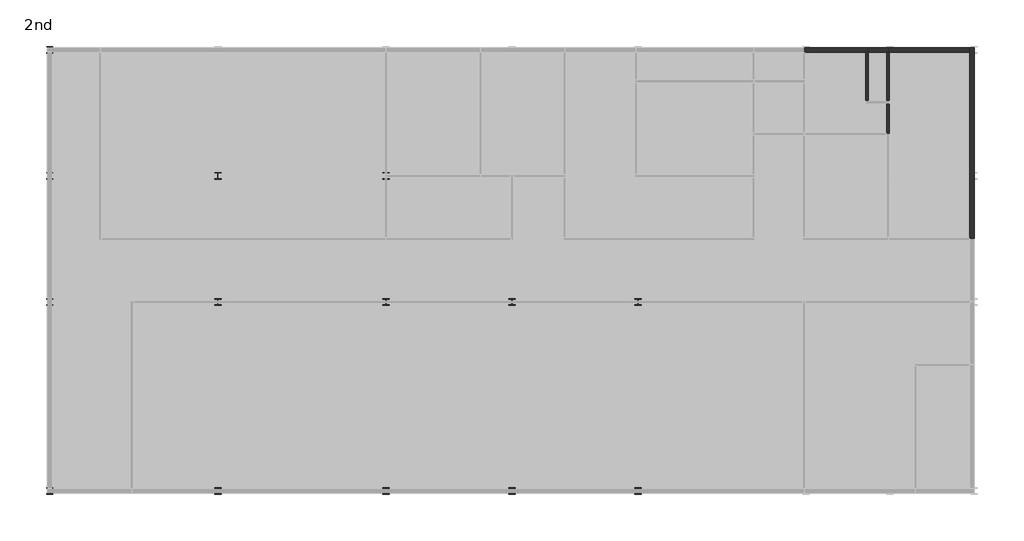
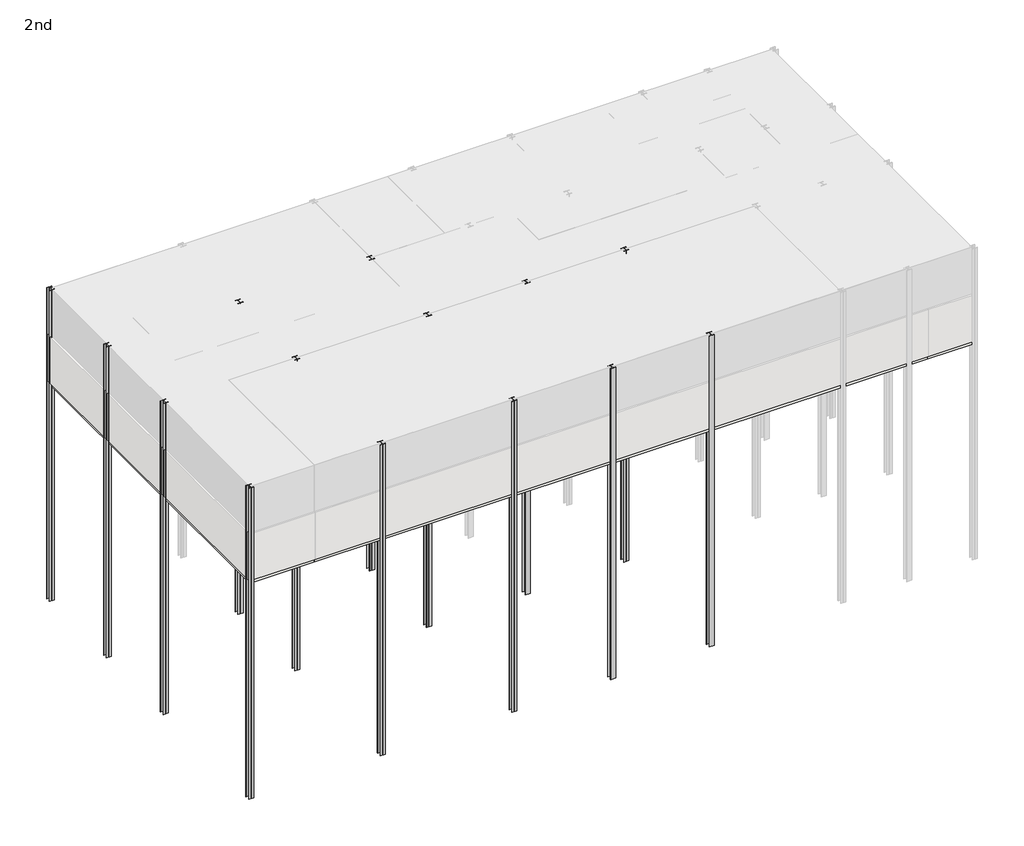
# One storey, part 2 of 3: 17 slabs, 14 columns, 7 walls.
"""IFC4 building model written with IfcOpenShell, lengths in millimetres."""

import ifcopenshell
import ifcopenshell.guid

model = None  # the IFC model being written
_history = None  # IfcOwnerHistory: only IFC2X3 demands one
_inside = {}  # id of a spatial element -> (the spatial element, [elements in it])
_under = {}  # id of a project, library or spatial element -> (it, [spatial elements below it])
_declared = {}  # id of a project -> (the project, [libraries it declares])
_typed = {}  # id of a type object -> (the type object, [elements of that type])
_made_of = {}  # id of a material, layer set ... -> (it, [elements and type objects made of it])


def new_model(schema):
    """Start an empty IFC model of exactly this schema.

    Asked for "IFC4X3", IfcOpenShell would pick the latest addendum, in which some entities
    have other attributes; the version numbers below select the first issue.
    IFC2X3 requires an IfcOwnerHistory on every rooted entity: one is made here for all.
    """
    global model, _history
    if schema == "IFC4X3":
        model = ifcopenshell.file(schema_version=(4, 3, 0, 0))
    else:
        model = ifcopenshell.file(schema=schema)
    _inside.clear()
    _under.clear()
    _declared.clear()
    _typed.clear()
    _made_of.clear()
    _history = None
    if model.schema == "IFC2X3":
        org = make("IfcOrganization", Name="unknown")
        user = make(
            "IfcPersonAndOrganization",
            ThePerson=make("IfcPerson", FamilyName="unknown"),
            TheOrganization=org,
        )
        app = make(
            "IfcApplication",
            ApplicationDeveloper=org,
            Version="unknown",
            ApplicationFullName="unknown",
            ApplicationIdentifier="unknown",
        )
        _history = make(
            "IfcOwnerHistory",
            OwningUser=user,
            OwningApplication=app,
            ChangeAction="ADDED",
            CreationDate=0,
        )
    return model


def make(cls, **values):
    """One entity of the class cls with the attributes given. An attribute that is None is left unset."""
    return model.create_entity(
        cls, **{name: value for name, value in values.items() if value is not None}
    )


def rooted(cls, **values):
    """An entity with a GlobalId (a new one), such as an element, a storey or a relation."""
    return make(cls, GlobalId=ifcopenshell.guid.new(), OwnerHistory=_history, **values)


def si_unit(unit_type, name, prefix=None):
    """IfcSIUnit, for example si_unit("LENGTHUNIT", "METRE", prefix="MILLI")."""
    return make("IfcSIUnit", UnitType=unit_type, Prefix=prefix, Name=name)


def assignment(units):
    """IfcUnitAssignment: the units of a project."""
    return None if units is None else make("IfcUnitAssignment", Units=units)


def point(xyz):
    """IfcCartesianPoint."""
    return None if xyz is None else make("IfcCartesianPoint", Coordinates=xyz)


def direction(xyz):
    """IfcDirection."""
    return None if xyz is None else make("IfcDirection", DirectionRatios=xyz)


def frame(location, z_axis=None, x_axis=None):
    """IfcAxis2Placement3D, a coordinate frame: its origin and axes. An axis left out is left unset."""
    return make(
        "IfcAxis2Placement3D",
        Location=point(location),
        Axis=direction(z_axis),
        RefDirection=direction(x_axis),
    )


def frame_2d(location, x_axis=None):
    """IfcAxis2Placement2D, a coordinate frame in the plane: its origin and x axis."""
    return make(
        "IfcAxis2Placement2D", Location=point(location), RefDirection=direction(x_axis)
    )


def origin():
    """The frame at (0, 0, 0) with its axes left unset."""
    return frame((0.0, 0.0, 0.0))


def origin_with_axes():
    """The frame at (0, 0, 0) with the z axis (0, 0, 1) and the x axis (1, 0, 0) written out."""
    return frame((0.0, 0.0, 0.0), z_axis=(0.0, 0.0, 1.0), x_axis=(1.0, 0.0, 0.0))


def place(relative_to, where):
    """IfcLocalPlacement: puts the frame where relative to a parent placement (None: the world)."""
    return make(
        "IfcLocalPlacement", PlacementRelTo=relative_to, RelativePlacement=where
    )


def context(
    kind, dimensions, precision=None, world=None, true_north=None, identifier=None
):
    """IfcGeometricRepresentationContext, for example the 3D "Model" context."""
    return make(
        "IfcGeometricRepresentationContext",
        ContextIdentifier=identifier,
        ContextType=kind,
        CoordinateSpaceDimension=dimensions,
        Precision=precision,
        WorldCoordinateSystem=world,
        TrueNorth=true_north,
    )


def project(units=None, contexts=None):
    """IfcProject with its units and contexts."""
    return rooted(
        "IfcProject",
        Name="project",
        RepresentationContexts=contexts,
        UnitsInContext=assignment(units),
    )


def spatial(cls, under=None, at=None, **own):
    """A site, building, storey or space (cls), placed at a placement, below another one or the project."""
    s = rooted(cls, ObjectPlacement=at, **own)
    if under is not None:
        _under.setdefault(under.id(), (under, []))[1].append(s)
    return s


def polyline(points):
    """IfcPolyline through the points."""
    return make("IfcPolyline", Points=[point(p) for p in points])


def circle_curve(where, radius):
    """IfcCircle in the frame where."""
    return make("IfcCircle", Position=where, Radius=radius)


def trimmed(basis, trim1, trim2, sense, master):
    """IfcTrimmedCurve: the piece of a basis curve between two trims."""
    return make(
        "IfcTrimmedCurve",
        BasisCurve=basis,
        Trim1=trim1,
        Trim2=trim2,
        SenseAgreement=sense,
        MasterRepresentation=master,
    )


def segment(curve, same_sense, transition):
    """IfcCompositeCurveSegment."""
    return make(
        "IfcCompositeCurveSegment",
        Transition=transition,
        SameSense=same_sense,
        ParentCurve=curve,
    )


def composite_curve(segments, self_intersect=None):
    """IfcCompositeCurve: segments joined end to end."""
    return make("IfcCompositeCurve", Segments=segments, SelfIntersect=self_intersect)


def outline(outer, holes=None, kind="AREA"):
    """IfcArbitraryClosedProfileDef: a profile drawn as a closed curve; with holes, ...WithVoids."""
    if holes is None:
        return make("IfcArbitraryClosedProfileDef", ProfileType=kind, OuterCurve=outer)
    return make(
        "IfcArbitraryProfileDefWithVoids",
        ProfileType=kind,
        OuterCurve=outer,
        InnerCurves=holes,
    )


def extrude(swept, where, along, depth):
    """IfcExtrudedAreaSolid: the profile swept, set in the frame where, extruded along a direction by depth."""
    return make(
        "IfcExtrudedAreaSolid",
        SweptArea=swept,
        Position=where,
        ExtrudedDirection=direction(along),
        Depth=depth,
    )


def faces_of(points, faces, orient=None, outer=None):
    """IfcFace entities. A face is a list of loops; a loop is a list of indices into points, from 0.

    orient and outer hold one flag for each loop. By default every Orientation is true, the
    first loop of a face is its IfcFaceOuterBound and the others are IfcFaceBound.
    """
    made = []
    for i, loops in enumerate(faces):
        bounds = []
        for j, loop in enumerate(loops):
            is_outer = j == 0 if outer is None else outer[i][j]
            bounds.append(
                make(
                    "IfcFaceOuterBound" if is_outer else "IfcFaceBound",
                    Bound=make("IfcPolyLoop", Polygon=[points[k] for k in loop]),
                    Orientation=True if orient is None else orient[i][j],
                )
            )
        made.append(make("IfcFace", Bounds=bounds))
    return made


def faceted_brep(points, faces, orient=None, outer=None, voids=None):
    """IfcFacetedBrep: a solid bounded by flat faces; with voids (closed shells), ...WithVoids."""
    shared = [point(p) for p in points]
    hull = make("IfcClosedShell", CfsFaces=faces_of(shared, faces, orient, outer))
    if voids is None:
        return make("IfcFacetedBrep", Outer=hull)
    return make(
        "IfcFacetedBrepWithVoids",
        Outer=hull,
        Voids=[
            make(cls, CfsFaces=faces_of(shared, fs, o, b)) for cls, fs, o, b in voids
        ],
    )


def shape(context_of_items, identifier, shape_type, items):
    """IfcShapeRepresentation: the items that make up one representation, for example the "Body"."""
    return make(
        "IfcShapeRepresentation",
        ContextOfItems=context_of_items,
        RepresentationIdentifier=identifier,
        RepresentationType=shape_type,
        Items=items,
    )


def made_of(thing, what):
    """Note that an element or type object is made of a material, layer set ...; save() writes the relation."""
    if what is not None:
        _made_of.setdefault(what.id(), (what, []))[1].append(thing)
    return thing


def element(
    cls,
    number,
    at=None,
    inside=None,
    cuts=None,
    type_object=None,
    material=None,
    context=None,
    identifier="Body",
    shape_type=None,
    held_by="IfcProductDefinitionShape",
    body=None,
    shapes=None,
    **own,
):
    """One element of the class cls, such as IfcWall. Its Tag is "e" and its number.

    at: its placement. inside: the storey or other place that contains it. cuts: it is an
    opening in that element (IfcRelVoidsElement). A single representation is given by context,
    identifier, shape_type and body (its items); several are given by shapes. held_by: the class
    of the entity that holds the representations. save() writes the other relations.
    """
    e = rooted(cls, Tag="e%d" % number, ObjectPlacement=at, **own)
    if body is not None:
        shapes = [shape(context, identifier, shape_type, body)]
    if shapes is not None:
        e.Representation = make(held_by, Representations=shapes)
    if inside is not None:
        _inside.setdefault(inside.id(), (inside, []))[1].append(e)
    if cuts is not None:
        rooted(
            "IfcRelVoidsElement", RelatingBuildingElement=cuts, RelatedOpeningElement=e
        )
    if type_object is not None:
        _typed.setdefault(type_object.id(), (type_object, []))[1].append(e)
    return made_of(e, material)


def aggregate(whole, parts):
    """IfcRelAggregates: a whole, such as a stair, and the parts it consists of."""
    return rooted("IfcRelAggregates", RelatingObject=whole, RelatedObjects=parts)


def save(model, path):
    """Write the relations noted so far, then the file.

    IfcRelAggregates (storeys below a building ...), IfcRelContainedInSpatialStructure (elements
    in a storey), IfcRelDefinesByType, IfcRelAssociatesMaterial and IfcRelDeclares: one each for
    every whole, place, type object, material and project.
    """
    for whole, parts in _under.values():
        aggregate(whole, parts)
    for where, things in _inside.values():
        rooted(
            "IfcRelContainedInSpatialStructure",
            RelatedElements=things,
            RelatingStructure=where,
        )
    for kind, things in _typed.values():
        rooted("IfcRelDefinesByType", RelatedObjects=things, RelatingType=kind)
    for what, things in _made_of.values():
        rooted("IfcRelAssociatesMaterial", RelatedObjects=things, RelatingMaterial=what)
    for by, libraries in _declared.values():
        rooted("IfcRelDeclares", RelatingContext=by, RelatedDefinitions=libraries)
    model.write(path)


model = new_model("IFC4")

# Units and contexts
model_context = context("Model", 3, world=origin())
ifc_project = project(units=[si_unit("LENGTHUNIT", "METRE", prefix="MILLI")], contexts=[model_context])

# Site, building, storey
site = spatial("IfcSite", under=ifc_project)
building = spatial("IfcBuilding", under=site)
storey = spatial("IfcBuildingStorey", under=building, Name="2nd", Elevation=14000.0)

# Columns
placement = place(None, origin())
element("IfcColumn", 1, ObjectType="UC-Universal Columns-Column : UC305x305x97", at=placement, inside=storey, context=model_context, shape_type="SweptSolid", body=[
    extrude(outline(composite_curve([segment(polyline([(156266.7520501, 152169.7081198), (156266.7520501, 152154.3081198), (156134.2520501, 152154.3081198)]), True, "CONTINUOUS"), segment(trimmed(circle_curve(frame_2d((156134.2520501, 152139.1081198)), 15.2), [point((156134.2520501, 152154.3081198))], [point((156119.0520501, 152139.1081198))], True, "CARTESIAN"), True, "CONTINUOUS"), segment(polyline([(156119.0520501, 152139.1081198), (156119.0520501, 151892.4081198)]), True, "CONTINUOUS"), segment(trimmed(circle_curve(frame_2d((156134.2520501, 151892.4081198)), 15.2), [point((156119.0520501, 151892.4081198))], [point((156134.2520501, 151877.2081198))], True, "CARTESIAN"), True, "CONTINUOUS"), segment(polyline([(156134.2520501, 151877.2081198), (156266.7520501, 151877.2081198), (156266.7520501, 151861.8081198), (155961.4520501, 151861.8081198), (155961.4520501, 151877.2081198), (156093.9520501, 151877.2081198)]), True, "CONTINUOUS"), segment(trimmed(circle_curve(frame_2d((156093.9520501, 151892.4081198)), 15.2), [point((156093.9520501, 151877.2081198))], [point((156109.1520501, 151892.4081198))], True, "CARTESIAN"), True, "CONTINUOUS"), segment(polyline([(156109.1520501, 151892.4081198), (156109.1520501, 152139.1081198)]), True, "CONTINUOUS"), segment(trimmed(circle_curve(frame_2d((156093.9520501, 152139.1081198)), 15.2), [point((156109.1520501, 152139.1081198))], [point((156093.9520501, 152154.3081198))], True, "CARTESIAN"), True, "CONTINUOUS"), segment(polyline([(156093.9520501, 152154.3081198), (155961.4520501, 152154.3081198), (155961.4520501, 152169.7081198), (156266.7520501, 152169.7081198)]), True, "CONTINUOUS")], self_intersect=False)), origin_with_axes(), (0.0, 0.0, 1.0), 20000.0),
])
element("IfcColumn", 2, ObjectType="UC-Universal Columns-Column : UC305x305x97", at=placement, inside=storey, context=model_context, shape_type="SweptSolid", body=[
    extrude(outline(composite_curve([segment(polyline([(156266.7520501, 146169.7081198), (156266.7520501, 146154.3081198), (156134.2520501, 146154.3081198)]), True, "CONTINUOUS"), segment(trimmed(circle_curve(frame_2d((156134.2520501, 146139.1081198)), 15.2), [point((156134.2520501, 146154.3081198))], [point((156119.0520501, 146139.1081198))], True, "CARTESIAN"), True, "CONTINUOUS"), segment(polyline([(156119.0520501, 146139.1081198), (156119.0520501, 145892.4081198)]), True, "CONTINUOUS"), segment(trimmed(circle_curve(frame_2d((156134.2520501, 145892.4081198)), 15.2), [point((156119.0520501, 145892.4081198))], [point((156134.2520501, 145877.2081198))], True, "CARTESIAN"), True, "CONTINUOUS"), segment(polyline([(156134.2520501, 145877.2081198), (156266.7520501, 145877.2081198), (156266.7520501, 145861.8081198), (155961.4520501, 145861.8081198), (155961.4520501, 145877.2081198), (156093.9520501, 145877.2081198)]), True, "CONTINUOUS"), segment(trimmed(circle_curve(frame_2d((156093.9520501, 145892.4081198)), 15.2), [point((156093.9520501, 145877.2081198))], [point((156109.1520501, 145892.4081198))], True, "CARTESIAN"), True, "CONTINUOUS"), segment(polyline([(156109.1520501, 145892.4081198), (156109.1520501, 146139.1081198)]), True, "CONTINUOUS"), segment(trimmed(circle_curve(frame_2d((156093.9520501, 146139.1081198)), 15.2), [point((156109.1520501, 146139.1081198))], [point((156093.9520501, 146154.3081198))], True, "CARTESIAN"), True, "CONTINUOUS"), segment(polyline([(156093.9520501, 146154.3081198), (155961.4520501, 146154.3081198), (155961.4520501, 146169.7081198), (156266.7520501, 146169.7081198)]), True, "CONTINUOUS")], self_intersect=False)), origin_with_axes(), (0.0, 0.0, 1.0), 20000.0),
])
element("IfcColumn", 3, ObjectType="UC-Universal Columns-Column : UC305x305x97", at=placement, inside=storey, context=model_context, shape_type="SweptSolid", body=[
    extrude(outline(composite_curve([segment(polyline([(156266.7520501, 140169.7081198), (156266.7520501, 140154.3081198), (156134.2520501, 140154.3081198)]), True, "CONTINUOUS"), segment(trimmed(circle_curve(frame_2d((156134.2520501, 140139.1081198)), 15.2), [point((156134.2520501, 140154.3081198))], [point((156119.0520501, 140139.1081198))], True, "CARTESIAN"), True, "CONTINUOUS"), segment(polyline([(156119.0520501, 140139.1081198), (156119.0520501, 139892.4081198)]), True, "CONTINUOUS"), segment(trimmed(circle_curve(frame_2d((156134.2520501, 139892.4081198)), 15.2), [point((156119.0520501, 139892.4081198))], [point((156134.2520501, 139877.2081198))], True, "CARTESIAN"), True, "CONTINUOUS"), segment(polyline([(156134.2520501, 139877.2081198), (156266.7520501, 139877.2081198), (156266.7520501, 139861.8081198), (155961.4520501, 139861.8081198), (155961.4520501, 139877.2081198), (156093.9520501, 139877.2081198)]), True, "CONTINUOUS"), segment(trimmed(circle_curve(frame_2d((156093.9520501, 139892.4081198)), 15.2), [point((156093.9520501, 139877.2081198))], [point((156109.1520501, 139892.4081198))], True, "CARTESIAN"), True, "CONTINUOUS"), segment(polyline([(156109.1520501, 139892.4081198), (156109.1520501, 140139.1081198)]), True, "CONTINUOUS"), segment(trimmed(circle_curve(frame_2d((156093.9520501, 140139.1081198)), 15.2), [point((156109.1520501, 140139.1081198))], [point((156093.9520501, 140154.3081198))], True, "CARTESIAN"), True, "CONTINUOUS"), segment(polyline([(156093.9520501, 140154.3081198), (155961.4520501, 140154.3081198), (155961.4520501, 140169.7081198), (156266.7520501, 140169.7081198)]), True, "CONTINUOUS")], self_intersect=False)), origin_with_axes(), (0.0, 0.0, 1.0), 20000.0),
])
element("IfcColumn", 4, ObjectType="UC-Universal Columns-Column : UC305x305x97", at=placement, inside=storey, context=model_context, shape_type="SweptSolid", body=[
    extrude(outline(composite_curve([segment(polyline([(156266.7520501, 131169.7081198), (156266.7520501, 131154.3081198), (156134.2520501, 131154.3081198)]), True, "CONTINUOUS"), segment(trimmed(circle_curve(frame_2d((156134.2520501, 131139.1081198)), 15.2), [point((156134.2520501, 131154.3081198))], [point((156119.0520501, 131139.1081198))], True, "CARTESIAN"), True, "CONTINUOUS"), segment(polyline([(156119.0520501, 131139.1081198), (156119.0520501, 130892.4081198)]), True, "CONTINUOUS"), segment(trimmed(circle_curve(frame_2d((156134.2520501, 130892.4081198)), 15.2), [point((156119.0520501, 130892.4081198))], [point((156134.2520501, 130877.2081198))], True, "CARTESIAN"), True, "CONTINUOUS"), segment(polyline([(156134.2520501, 130877.2081198), (156266.7520501, 130877.2081198), (156266.7520501, 130861.8081198), (155961.4520501, 130861.8081198), (155961.4520501, 130877.2081198), (156093.9520501, 130877.2081198)]), True, "CONTINUOUS"), segment(trimmed(circle_curve(frame_2d((156093.9520501, 130892.4081198)), 15.2), [point((156093.9520501, 130877.2081198))], [point((156109.1520501, 130892.4081198))], True, "CARTESIAN"), True, "CONTINUOUS"), segment(polyline([(156109.1520501, 130892.4081198), (156109.1520501, 131139.1081198)]), True, "CONTINUOUS"), segment(trimmed(circle_curve(frame_2d((156093.9520501, 131139.1081198)), 15.2), [point((156109.1520501, 131139.1081198))], [point((156093.9520501, 131154.3081198))], True, "CARTESIAN"), True, "CONTINUOUS"), segment(polyline([(156093.9520501, 131154.3081198), (155961.4520501, 131154.3081198), (155961.4520501, 131169.7081198), (156266.7520501, 131169.7081198)]), True, "CONTINUOUS")], self_intersect=False)), origin_with_axes(), (0.0, 0.0, 1.0), 20000.0),
])
element("IfcColumn", 5, ObjectType="UC-Universal Columns-Column : UC305x305x97", at=placement, inside=storey, context=model_context, shape_type="SweptSolid", body=[
    extrude(outline(composite_curve([segment(polyline([(164266.7520501, 146169.7081198), (164266.7520501, 146154.3081198), (164134.2520501, 146154.3081198)]), True, "CONTINUOUS"), segment(trimmed(circle_curve(frame_2d((164134.2520501, 146139.1081198)), 15.2), [point((164134.2520501, 146154.3081198))], [point((164119.0520501, 146139.1081198))], True, "CARTESIAN"), True, "CONTINUOUS"), segment(polyline([(164119.0520501, 146139.1081198), (164119.0520501, 145892.4081198)]), True, "CONTINUOUS"), segment(trimmed(circle_curve(frame_2d((164134.2520501, 145892.4081198)), 15.2), [point((164119.0520501, 145892.4081198))], [point((164134.2520501, 145877.2081198))], True, "CARTESIAN"), True, "CONTINUOUS"), segment(polyline([(164134.2520501, 145877.2081198), (164266.7520501, 145877.2081198), (164266.7520501, 145861.8081198), (163961.4520501, 145861.8081198), (163961.4520501, 145877.2081198), (164093.9520501, 145877.2081198)]), True, "CONTINUOUS"), segment(trimmed(circle_curve(frame_2d((164093.9520501, 145892.4081198)), 15.2), [point((164093.9520501, 145877.2081198))], [point((164109.1520501, 145892.4081198))], True, "CARTESIAN"), True, "CONTINUOUS"), segment(polyline([(164109.1520501, 145892.4081198), (164109.1520501, 146139.1081198)]), True, "CONTINUOUS"), segment(trimmed(circle_curve(frame_2d((164093.9520501, 146139.1081198)), 15.2), [point((164109.1520501, 146139.1081198))], [point((164093.9520501, 146154.3081198))], True, "CARTESIAN"), True, "CONTINUOUS"), segment(polyline([(164093.9520501, 146154.3081198), (163961.4520501, 146154.3081198), (163961.4520501, 146169.7081198), (164266.7520501, 146169.7081198)]), True, "CONTINUOUS")], self_intersect=False)), origin_with_axes(), (0.0, 0.0, 1.0), 20000.0),
])
element("IfcColumn", 6, ObjectType="UC-Universal Columns-Column : UC305x305x97", at=placement, inside=storey, context=model_context, shape_type="SweptSolid", body=[
    extrude(outline(composite_curve([segment(polyline([(164266.7520501, 140169.7081198), (164266.7520501, 140154.3081198), (164134.2520501, 140154.3081198)]), True, "CONTINUOUS"), segment(trimmed(circle_curve(frame_2d((164134.2520501, 140139.1081198)), 15.2), [point((164134.2520501, 140154.3081198))], [point((164119.0520501, 140139.1081198))], True, "CARTESIAN"), True, "CONTINUOUS"), segment(polyline([(164119.0520501, 140139.1081198), (164119.0520501, 139892.4081198)]), True, "CONTINUOUS"), segment(trimmed(circle_curve(frame_2d((164134.2520501, 139892.4081198)), 15.2), [point((164119.0520501, 139892.4081198))], [point((164134.2520501, 139877.2081198))], True, "CARTESIAN"), True, "CONTINUOUS"), segment(polyline([(164134.2520501, 139877.2081198), (164266.7520501, 139877.2081198), (164266.7520501, 139861.8081198), (163961.4520501, 139861.8081198), (163961.4520501, 139877.2081198), (164093.9520501, 139877.2081198)]), True, "CONTINUOUS"), segment(trimmed(circle_curve(frame_2d((164093.9520501, 139892.4081198)), 15.2), [point((164093.9520501, 139877.2081198))], [point((164109.1520501, 139892.4081198))], True, "CARTESIAN"), True, "CONTINUOUS"), segment(polyline([(164109.1520501, 139892.4081198), (164109.1520501, 140139.1081198)]), True, "CONTINUOUS"), segment(trimmed(circle_curve(frame_2d((164093.9520501, 140139.1081198)), 15.2), [point((164109.1520501, 140139.1081198))], [point((164093.9520501, 140154.3081198))], True, "CARTESIAN"), True, "CONTINUOUS"), segment(polyline([(164093.9520501, 140154.3081198), (163961.4520501, 140154.3081198), (163961.4520501, 140169.7081198), (164266.7520501, 140169.7081198)]), True, "CONTINUOUS")], self_intersect=False)), origin_with_axes(), (0.0, 0.0, 1.0), 20000.0),
])
element("IfcColumn", 7, ObjectType="UC-Universal Columns-Column : UC305x305x97", at=placement, inside=storey, context=model_context, shape_type="SweptSolid", body=[
    extrude(outline(composite_curve([segment(polyline([(164266.7520501, 131169.7081198), (164266.7520501, 131154.3081198), (164134.2520501, 131154.3081198)]), True, "CONTINUOUS"), segment(trimmed(circle_curve(frame_2d((164134.2520501, 131139.1081198)), 15.2), [point((164134.2520501, 131154.3081198))], [point((164119.0520501, 131139.1081198))], True, "CARTESIAN"), True, "CONTINUOUS"), segment(polyline([(164119.0520501, 131139.1081198), (164119.0520501, 130892.4081198)]), True, "CONTINUOUS"), segment(trimmed(circle_curve(frame_2d((164134.2520501, 130892.4081198)), 15.2), [point((164119.0520501, 130892.4081198))], [point((164134.2520501, 130877.2081198))], True, "CARTESIAN"), True, "CONTINUOUS"), segment(polyline([(164134.2520501, 130877.2081198), (164266.7520501, 130877.2081198), (164266.7520501, 130861.8081198), (163961.4520501, 130861.8081198), (163961.4520501, 130877.2081198), (164093.9520501, 130877.2081198)]), True, "CONTINUOUS"), segment(trimmed(circle_curve(frame_2d((164093.9520501, 130892.4081198)), 15.2), [point((164093.9520501, 130877.2081198))], [point((164109.1520501, 130892.4081198))], True, "CARTESIAN"), True, "CONTINUOUS"), segment(polyline([(164109.1520501, 130892.4081198), (164109.1520501, 131139.1081198)]), True, "CONTINUOUS"), segment(trimmed(circle_curve(frame_2d((164093.9520501, 131139.1081198)), 15.2), [point((164109.1520501, 131139.1081198))], [point((164093.9520501, 131154.3081198))], True, "CARTESIAN"), True, "CONTINUOUS"), segment(polyline([(164093.9520501, 131154.3081198), (163961.4520501, 131154.3081198), (163961.4520501, 131169.7081198), (164266.7520501, 131169.7081198)]), True, "CONTINUOUS")], self_intersect=False)), origin_with_axes(), (0.0, 0.0, 1.0), 20000.0),
])
element("IfcColumn", 8, ObjectType="UC-Universal Columns-Column : UC305x305x97", at=placement, inside=storey, context=model_context, shape_type="SweptSolid", body=[
    extrude(outline(composite_curve([segment(polyline([(172266.7520501, 146169.7081198), (172266.7520501, 146154.3081198), (172134.2520501, 146154.3081198)]), True, "CONTINUOUS"), segment(trimmed(circle_curve(frame_2d((172134.2520501, 146139.1081198)), 15.2), [point((172134.2520501, 146154.3081198))], [point((172119.0520501, 146139.1081198))], True, "CARTESIAN"), True, "CONTINUOUS"), segment(polyline([(172119.0520501, 146139.1081198), (172119.0520501, 145892.4081198)]), True, "CONTINUOUS"), segment(trimmed(circle_curve(frame_2d((172134.2520501, 145892.4081198)), 15.2), [point((172119.0520501, 145892.4081198))], [point((172134.2520501, 145877.2081198))], True, "CARTESIAN"), True, "CONTINUOUS"), segment(polyline([(172134.2520501, 145877.2081198), (172266.7520501, 145877.2081198), (172266.7520501, 145861.8081198), (171961.4520501, 145861.8081198), (171961.4520501, 145877.2081198), (172093.9520501, 145877.2081198)]), True, "CONTINUOUS"), segment(trimmed(circle_curve(frame_2d((172093.9520501, 145892.4081198)), 15.2), [point((172093.9520501, 145877.2081198))], [point((172109.1520501, 145892.4081198))], True, "CARTESIAN"), True, "CONTINUOUS"), segment(polyline([(172109.1520501, 145892.4081198), (172109.1520501, 146139.1081198)]), True, "CONTINUOUS"), segment(trimmed(circle_curve(frame_2d((172093.9520501, 146139.1081198)), 15.2), [point((172109.1520501, 146139.1081198))], [point((172093.9520501, 146154.3081198))], True, "CARTESIAN"), True, "CONTINUOUS"), segment(polyline([(172093.9520501, 146154.3081198), (171961.4520501, 146154.3081198), (171961.4520501, 146169.7081198), (172266.7520501, 146169.7081198)]), True, "CONTINUOUS")], self_intersect=False)), origin_with_axes(), (0.0, 0.0, 1.0), 20000.0),
])
element("IfcColumn", 9, ObjectType="UC-Universal Columns-Column : UC305x305x97", at=placement, inside=storey, context=model_context, shape_type="SweptSolid", body=[
    extrude(outline(composite_curve([segment(polyline([(172266.7520501, 140169.7081198), (172266.7520501, 140154.3081198), (172134.2520501, 140154.3081198)]), True, "CONTINUOUS"), segment(trimmed(circle_curve(frame_2d((172134.2520501, 140139.1081198)), 15.2), [point((172134.2520501, 140154.3081198))], [point((172119.0520501, 140139.1081198))], True, "CARTESIAN"), True, "CONTINUOUS"), segment(polyline([(172119.0520501, 140139.1081198), (172119.0520501, 139892.4081198)]), True, "CONTINUOUS"), segment(trimmed(circle_curve(frame_2d((172134.2520501, 139892.4081198)), 15.2), [point((172119.0520501, 139892.4081198))], [point((172134.2520501, 139877.2081198))], True, "CARTESIAN"), True, "CONTINUOUS"), segment(polyline([(172134.2520501, 139877.2081198), (172266.7520501, 139877.2081198), (172266.7520501, 139861.8081198), (171961.4520501, 139861.8081198), (171961.4520501, 139877.2081198), (172093.9520501, 139877.2081198)]), True, "CONTINUOUS"), segment(trimmed(circle_curve(frame_2d((172093.9520501, 139892.4081198)), 15.2), [point((172093.9520501, 139877.2081198))], [point((172109.1520501, 139892.4081198))], True, "CARTESIAN"), True, "CONTINUOUS"), segment(polyline([(172109.1520501, 139892.4081198), (172109.1520501, 140139.1081198)]), True, "CONTINUOUS"), segment(trimmed(circle_curve(frame_2d((172093.9520501, 140139.1081198)), 15.2), [point((172109.1520501, 140139.1081198))], [point((172093.9520501, 140154.3081198))], True, "CARTESIAN"), True, "CONTINUOUS"), segment(polyline([(172093.9520501, 140154.3081198), (171961.4520501, 140154.3081198), (171961.4520501, 140169.7081198), (172266.7520501, 140169.7081198)]), True, "CONTINUOUS")], self_intersect=False)), origin_with_axes(), (0.0, 0.0, 1.0), 20000.0),
])
element("IfcColumn", 10, ObjectType="UC-Universal Columns-Column : UC305x305x97", at=placement, inside=storey, context=model_context, shape_type="SweptSolid", body=[
    extrude(outline(composite_curve([segment(polyline([(172266.7520501, 131169.7081198), (172266.7520501, 131154.3081198), (172134.2520501, 131154.3081198)]), True, "CONTINUOUS"), segment(trimmed(circle_curve(frame_2d((172134.2520501, 131139.1081198)), 15.2), [point((172134.2520501, 131154.3081198))], [point((172119.0520501, 131139.1081198))], True, "CARTESIAN"), True, "CONTINUOUS"), segment(polyline([(172119.0520501, 131139.1081198), (172119.0520501, 130892.4081198)]), True, "CONTINUOUS"), segment(trimmed(circle_curve(frame_2d((172134.2520501, 130892.4081198)), 15.2), [point((172119.0520501, 130892.4081198))], [point((172134.2520501, 130877.2081198))], True, "CARTESIAN"), True, "CONTINUOUS"), segment(polyline([(172134.2520501, 130877.2081198), (172266.7520501, 130877.2081198), (172266.7520501, 130861.8081198), (171961.4520501, 130861.8081198), (171961.4520501, 130877.2081198), (172093.9520501, 130877.2081198)]), True, "CONTINUOUS"), segment(trimmed(circle_curve(frame_2d((172093.9520501, 130892.4081198)), 15.2), [point((172093.9520501, 130877.2081198))], [point((172109.1520501, 130892.4081198))], True, "CARTESIAN"), True, "CONTINUOUS"), segment(polyline([(172109.1520501, 130892.4081198), (172109.1520501, 131139.1081198)]), True, "CONTINUOUS"), segment(trimmed(circle_curve(frame_2d((172093.9520501, 131139.1081198)), 15.2), [point((172109.1520501, 131139.1081198))], [point((172093.9520501, 131154.3081198))], True, "CARTESIAN"), True, "CONTINUOUS"), segment(polyline([(172093.9520501, 131154.3081198), (171961.4520501, 131154.3081198), (171961.4520501, 131169.7081198), (172266.7520501, 131169.7081198)]), True, "CONTINUOUS")], self_intersect=False)), origin_with_axes(), (0.0, 0.0, 1.0), 20000.0),
])
element("IfcColumn", 11, ObjectType="UC-Universal Columns-Column : UC305x305x97", at=placement, inside=storey, context=model_context, shape_type="SweptSolid", body=[
    extrude(outline(composite_curve([segment(polyline([(178266.7520501, 140169.7081198), (178266.7520501, 140154.3081198), (178134.2520501, 140154.3081198)]), True, "CONTINUOUS"), segment(trimmed(circle_curve(frame_2d((178134.2520501, 140139.1081198)), 15.2), [point((178134.2520501, 140154.3081198))], [point((178119.0520501, 140139.1081198))], True, "CARTESIAN"), True, "CONTINUOUS"), segment(polyline([(178119.0520501, 140139.1081198), (178119.0520501, 139892.4081198)]), True, "CONTINUOUS"), segment(trimmed(circle_curve(frame_2d((178134.2520501, 139892.4081198)), 15.2), [point((178119.0520501, 139892.4081198))], [point((178134.2520501, 139877.2081198))], True, "CARTESIAN"), True, "CONTINUOUS"), segment(polyline([(178134.2520501, 139877.2081198), (178266.7520501, 139877.2081198), (178266.7520501, 139861.8081198), (177961.4520501, 139861.8081198), (177961.4520501, 139877.2081198), (178093.9520501, 139877.2081198)]), True, "CONTINUOUS"), segment(trimmed(circle_curve(frame_2d((178093.9520501, 139892.4081198)), 15.2), [point((178093.9520501, 139877.2081198))], [point((178109.1520501, 139892.4081198))], True, "CARTESIAN"), True, "CONTINUOUS"), segment(polyline([(178109.1520501, 139892.4081198), (178109.1520501, 140139.1081198)]), True, "CONTINUOUS"), segment(trimmed(circle_curve(frame_2d((178093.9520501, 140139.1081198)), 15.2), [point((178109.1520501, 140139.1081198))], [point((178093.9520501, 140154.3081198))], True, "CARTESIAN"), True, "CONTINUOUS"), segment(polyline([(178093.9520501, 140154.3081198), (177961.4520501, 140154.3081198), (177961.4520501, 140169.7081198), (178266.7520501, 140169.7081198)]), True, "CONTINUOUS")], self_intersect=False)), origin_with_axes(), (0.0, 0.0, 1.0), 20000.0),
])
element("IfcColumn", 12, ObjectType="UC-Universal Columns-Column : UC305x305x97", at=placement, inside=storey, context=model_context, shape_type="SweptSolid", body=[
    extrude(outline(composite_curve([segment(polyline([(178266.7520501, 131169.7081198), (178266.7520501, 131154.3081198), (178134.2520501, 131154.3081198)]), True, "CONTINUOUS"), segment(trimmed(circle_curve(frame_2d((178134.2520501, 131139.1081198)), 15.2), [point((178134.2520501, 131154.3081198))], [point((178119.0520501, 131139.1081198))], True, "CARTESIAN"), True, "CONTINUOUS"), segment(polyline([(178119.0520501, 131139.1081198), (178119.0520501, 130892.4081198)]), True, "CONTINUOUS"), segment(trimmed(circle_curve(frame_2d((178134.2520501, 130892.4081198)), 15.2), [point((178119.0520501, 130892.4081198))], [point((178134.2520501, 130877.2081198))], True, "CARTESIAN"), True, "CONTINUOUS"), segment(polyline([(178134.2520501, 130877.2081198), (178266.7520501, 130877.2081198), (178266.7520501, 130861.8081198), (177961.4520501, 130861.8081198), (177961.4520501, 130877.2081198), (178093.9520501, 130877.2081198)]), True, "CONTINUOUS"), segment(trimmed(circle_curve(frame_2d((178093.9520501, 130892.4081198)), 15.2), [point((178093.9520501, 130877.2081198))], [point((178109.1520501, 130892.4081198))], True, "CARTESIAN"), True, "CONTINUOUS"), segment(polyline([(178109.1520501, 130892.4081198), (178109.1520501, 131139.1081198)]), True, "CONTINUOUS"), segment(trimmed(circle_curve(frame_2d((178093.9520501, 131139.1081198)), 15.2), [point((178109.1520501, 131139.1081198))], [point((178093.9520501, 131154.3081198))], True, "CARTESIAN"), True, "CONTINUOUS"), segment(polyline([(178093.9520501, 131154.3081198), (177961.4520501, 131154.3081198), (177961.4520501, 131169.7081198), (178266.7520501, 131169.7081198)]), True, "CONTINUOUS")], self_intersect=False)), origin_with_axes(), (0.0, 0.0, 1.0), 20000.0),
])
element("IfcColumn", 13, ObjectType="UC-Universal Columns-Column : UC305x305x97", at=placement, inside=storey, context=model_context, shape_type="SweptSolid", body=[
    extrude(outline(composite_curve([segment(polyline([(184266.7520501, 140169.7081198), (184266.7520501, 140154.3081198), (184134.2520501, 140154.3081198)]), True, "CONTINUOUS"), segment(trimmed(circle_curve(frame_2d((184134.2520501, 140139.1081198)), 15.2), [point((184134.2520501, 140154.3081198))], [point((184119.0520501, 140139.1081198))], True, "CARTESIAN"), True, "CONTINUOUS"), segment(polyline([(184119.0520501, 140139.1081198), (184119.0520501, 139892.4081198)]), True, "CONTINUOUS"), segment(trimmed(circle_curve(frame_2d((184134.2520501, 139892.4081198)), 15.2), [point((184119.0520501, 139892.4081198))], [point((184134.2520501, 139877.2081198))], True, "CARTESIAN"), True, "CONTINUOUS"), segment(polyline([(184134.2520501, 139877.2081198), (184266.7520501, 139877.2081198), (184266.7520501, 139861.8081198), (183961.4520501, 139861.8081198), (183961.4520501, 139877.2081198), (184093.9520501, 139877.2081198)]), True, "CONTINUOUS"), segment(trimmed(circle_curve(frame_2d((184093.9520501, 139892.4081198)), 15.2), [point((184093.9520501, 139877.2081198))], [point((184109.1520501, 139892.4081198))], True, "CARTESIAN"), True, "CONTINUOUS"), segment(polyline([(184109.1520501, 139892.4081198), (184109.1520501, 140139.1081198)]), True, "CONTINUOUS"), segment(trimmed(circle_curve(frame_2d((184093.9520501, 140139.1081198)), 15.2), [point((184109.1520501, 140139.1081198))], [point((184093.9520501, 140154.3081198))], True, "CARTESIAN"), True, "CONTINUOUS"), segment(polyline([(184093.9520501, 140154.3081198), (183961.4520501, 140154.3081198), (183961.4520501, 140169.7081198), (184266.7520501, 140169.7081198)]), True, "CONTINUOUS")], self_intersect=False)), origin_with_axes(), (0.0, 0.0, 1.0), 20000.0),
])
element("IfcColumn", 14, ObjectType="UC-Universal Columns-Column : UC305x305x97", at=placement, inside=storey, context=model_context, shape_type="SweptSolid", body=[
    extrude(outline(composite_curve([segment(polyline([(184266.7520501, 131169.7081198), (184266.7520501, 131154.3081198), (184134.2520501, 131154.3081198)]), True, "CONTINUOUS"), segment(trimmed(circle_curve(frame_2d((184134.2520501, 131139.1081198)), 15.2), [point((184134.2520501, 131154.3081198))], [point((184119.0520501, 131139.1081198))], True, "CARTESIAN"), True, "CONTINUOUS"), segment(polyline([(184119.0520501, 131139.1081198), (184119.0520501, 130892.4081198)]), True, "CONTINUOUS"), segment(trimmed(circle_curve(frame_2d((184134.2520501, 130892.4081198)), 15.2), [point((184119.0520501, 130892.4081198))], [point((184134.2520501, 130877.2081198))], True, "CARTESIAN"), True, "CONTINUOUS"), segment(polyline([(184134.2520501, 130877.2081198), (184266.7520501, 130877.2081198), (184266.7520501, 130861.8081198), (183961.4520501, 130861.8081198), (183961.4520501, 130877.2081198), (184093.9520501, 130877.2081198)]), True, "CONTINUOUS"), segment(trimmed(circle_curve(frame_2d((184093.9520501, 130892.4081198)), 15.2), [point((184093.9520501, 130877.2081198))], [point((184109.1520501, 130892.4081198))], True, "CARTESIAN"), True, "CONTINUOUS"), segment(polyline([(184109.1520501, 130892.4081198), (184109.1520501, 131139.1081198)]), True, "CONTINUOUS"), segment(trimmed(circle_curve(frame_2d((184093.9520501, 131139.1081198)), 15.2), [point((184109.1520501, 131139.1081198))], [point((184093.9520501, 131154.3081198))], True, "CARTESIAN"), True, "CONTINUOUS"), segment(polyline([(184093.9520501, 131154.3081198), (183961.4520501, 131154.3081198), (183961.4520501, 131169.7081198), (184266.7520501, 131169.7081198)]), True, "CONTINUOUS")], self_intersect=False)), origin_with_axes(), (0.0, 0.0, 1.0), 20000.0),
])

# Slabs
element("IfcSlab", 15, ObjectType="Floor_Timber_22Cbd-225Joist", at=placement, inside=storey, context=model_context, shape_type="SweptSolid", body=[
    extrude(outline(polyline([(160014.1020501, 140015.7581198), (192014.1020501, 140015.7581198), (192014.1020501, 131015.7581198), (160014.1020501, 131015.7581198), (160014.1020501, 140015.7581198)])), frame((0.0, 0.0, 13753.0), z_axis=(0.0, 0.0, 1.0), x_axis=(1.0, 0.0, 0.0)), (0.0, 0.0, 1.0), 247.0),
])
element("IfcSlab", 16, ObjectType="Floor_Timber_22Cbd-225Joist", at=placement, inside=storey, context=model_context, shape_type="SweptSolid", body=[
    extrude(outline(polyline([(158514.1020501, 152015.7581198), (172114.1020501, 152015.7581198), (172114.1020501, 143015.7581198), (158514.1020501, 143015.7581198), (158514.1020501, 152015.7581198)])), frame((0.0, 0.0, 13753.0), z_axis=(0.0, 0.0, 1.0), x_axis=(1.0, 0.0, 0.0)), (0.0, 0.0, 1.0), 247.0),
])
element("IfcSlab", 17, ObjectType="Floor_Timber_22Cbd-225Joist", at=placement, inside=storey, context=model_context, shape_type="SweptSolid", body=[
    extrude(outline(polyline([(172114.1020501, 146015.7581198), (172114.1020501, 152015.7581198), (176614.1020501, 152015.7581198), (176614.1020501, 146015.7581198), (172114.1020501, 146015.7581198)])), frame((0.0, 0.0, 13753.0), z_axis=(0.0, 0.0, 1.0), x_axis=(1.0, 0.0, 0.0)), (0.0, 0.0, 1.0), 247.0),
])
element("IfcSlab", 18, ObjectType="Floor_Timber_22Cbd-225Joist", at=placement, inside=storey, context=model_context, shape_type="SweptSolid", body=[
    extrude(outline(polyline([(192014.1020501, 143015.7581198), (192014.1020501, 148015.7581198), (196014.1020501, 148015.7581198), (196014.1020501, 143015.7581198), (192014.1020501, 143015.7581198)])), frame((0.0, 0.0, 13753.0), z_axis=(0.0, 0.0, 1.0), x_axis=(1.0, 0.0, 0.0)), (0.0, 0.0, 1.0), 247.0),
])
element("IfcSlab", 19, ObjectType="Floor_Timber_22Cbd-225Joist", at=placement, inside=storey, context=model_context, shape_type="SweptSolid", body=[
    extrude(outline(polyline([(200014.1020501, 143015.7581198), (196014.1020501, 143015.7581198), (196014.1020501, 152015.7581198), (200014.1020501, 152015.7581198), (200014.1020501, 143015.7581198)])), frame((0.0, 0.0, 13753.0), z_axis=(0.0, 0.0, 1.0), x_axis=(1.0, 0.0, 0.0)), (0.0, 0.0, 1.0), 247.0),
])
element("IfcSlab", 20, ObjectType="Floor_Timber_22Cbd-225Joist", at=placement, inside=storey, context=model_context, shape_type="SweptSolid", body=[
    extrude(outline(polyline([(176614.1020501, 146015.7581198), (176614.1020501, 152015.7581198), (180614.1020501, 152015.7581198), (180614.1020501, 146015.7581198), (176614.1020501, 146015.7581198)])), frame((0.0, 0.0, 13753.0), z_axis=(0.0, 0.0, 1.0), x_axis=(1.0, 0.0, 0.0)), (0.0, 0.0, 1.0), 247.0),
])
element("IfcSlab", 21, ObjectType="Floor_Timber_22Cbd-225Joist", at=placement, inside=storey, context=model_context, shape_type="SweptSolid", body=[
    extrude(outline(polyline([(172114.1020501, 143015.7581198), (172114.1020501, 146015.7581198), (178114.1020501, 146015.7581198), (178114.1020501, 143015.7581198), (172114.1020501, 143015.7581198)])), frame((0.0, 0.0, 13753.0), z_axis=(0.0, 0.0, 1.0), x_axis=(1.0, 0.0, 0.0)), (0.0, 0.0, 1.0), 247.0),
])
element("IfcSlab", 22, ObjectType="Floor_Timber_22Cbd-225Joist", at=placement, inside=storey, context=model_context, shape_type="SweptSolid", body=[
    extrude(outline(polyline([(189614.1020501, 150515.7581198), (189614.1020501, 152015.7581198), (192014.1020501, 152015.7581198), (192014.1020501, 150515.7581198), (189614.1020501, 150515.7581198)])), frame((0.0, 0.0, 13753.0), z_axis=(0.0, 0.0, 1.0), x_axis=(1.0, 0.0, 0.0)), (0.0, 0.0, 1.0), 247.0),
])
element("IfcSlab", 23, ObjectType="Floor_Timber_22Cbd-225Joist", at=placement, inside=storey, context=model_context, shape_type="SweptSolid", body=[
    extrude(outline(polyline([(200014.1020501, 140015.7581198), (160014.1020501, 140015.7581198), (160014.1020501, 131015.7581198), (156114.1020501, 131015.7581198), (156114.1020501, 152015.7581198), (158514.1020501, 152015.7581198), (158514.1020501, 143015.7581198), (178114.1020501, 143015.7581198), (178114.1020501, 146015.7581198), (180614.1020501, 146015.7581198), (180614.1020501, 143015.7581198), (189614.1020501, 143015.7581198), (189614.1020501, 148015.7581198), (192014.1020501, 148015.7581198), (192014.1020501, 143015.7581198), (200014.1020501, 143015.7581198), (200014.1020501, 140015.7581198)])), frame((0.0, 0.0, 13753.0), z_axis=(0.0, 0.0, 1.0), x_axis=(1.0, 0.0, 0.0)), (0.0, 0.0, 1.0), 247.0),
])
element("IfcSlab", 24, ObjectType="Floor_Timber_22Cbd-225Joist", at=placement, inside=storey, context=model_context, shape_type="SweptSolid", body=[
    extrude(outline(polyline([(189614.1020501, 148015.7581198), (189614.1020501, 150515.7581198), (192014.1020501, 150515.7581198), (192014.1020501, 148015.7581198), (189614.1020501, 148015.7581198)])), frame((0.0, 0.0, 13753.0), z_axis=(0.0, 0.0, 1.0), x_axis=(1.0, 0.0, 0.0)), (0.0, 0.0, 1.0), 247.0),
])
element("IfcSlab", 25, ObjectType="Floor_Timber_22Cbd-225Joist", at=placement, inside=storey, context=model_context, shape_type="SweptSolid", body=[
    extrude(outline(polyline([(184014.1020501, 152015.7581198), (189614.1020501, 152015.7581198), (189614.1020501, 150515.7581198), (184014.1020501, 150515.7581198), (184014.1020501, 152015.7581198)])), frame((0.0, 0.0, 13753.0), z_axis=(0.0, 0.0, 1.0), x_axis=(1.0, 0.0, 0.0)), (0.0, 0.0, 1.0), 247.0),
])
element("IfcSlab", 26, ObjectType="Floor_Timber_22Cbd-225Joist", at=placement, inside=storey, context=model_context, shape_type="SweptSolid", body=[
    extrude(outline(polyline([(189614.1020501, 143015.7581198), (180614.1020501, 143015.7581198), (180614.1020501, 152015.7581198), (184014.1020501, 152015.7581198), (184014.1020501, 146015.7581198), (189614.1020501, 146015.7581198), (189614.1020501, 143015.7581198)])), frame((0.0, 0.0, 13753.0), z_axis=(0.0, 0.0, 1.0), x_axis=(1.0, 0.0, 0.0)), (0.0, 0.0, 1.0), 247.0),
])
element("IfcSlab", 27, ObjectType="Floor_Timber_22Cbd-225Joist", at=placement, inside=storey, context=model_context, shape_type="SweptSolid", body=[
    extrude(outline(polyline([(184014.1020501, 150515.7581198), (189614.1020501, 150515.7581198), (189614.1020501, 146015.7581198), (184014.1020501, 146015.7581198), (184014.1020501, 150515.7581198)])), frame((0.0, 0.0, 13753.0), z_axis=(0.0, 0.0, 1.0), x_axis=(1.0, 0.0, 0.0)), (0.0, 0.0, 1.0), 247.0),
])
element("IfcSlab", 28, ObjectType="Floor_Timber_22Cbd-225Joist", at=placement, inside=storey, context=model_context, shape_type="SweptSolid", body=[
    extrude(outline(polyline([(192014.1020501, 131015.7581198), (192014.1020501, 140015.7581198), (200014.1020501, 140015.7581198), (200014.1020501, 137015.7581198), (197314.1020501, 137015.7581198), (197314.1020501, 131015.7581198), (192014.1020501, 131015.7581198)])), frame((0.0, 0.0, 13753.0), z_axis=(0.0, 0.0, 1.0), x_axis=(1.0, 0.0, 0.0)), (0.0, 0.0, 1.0), 247.0),
])
element("IfcSlab", 29, ObjectType="Floor_Timber_22Cbd-225Joist", at=placement, inside=storey, context=model_context, shape_type="SweptSolid", body=[
    extrude(outline(polyline([(200014.1020501, 137015.7581198), (200014.1020501, 131015.7581198), (197314.1020501, 131015.7581198), (197314.1020501, 137015.7581198), (200014.1020501, 137015.7581198)])), frame((0.0, 0.0, 13753.0), z_axis=(0.0, 0.0, 1.0), x_axis=(1.0, 0.0, 0.0)), (0.0, 0.0, 1.0), 247.0),
])
element("IfcSlab", 30, ObjectType="Floor_Timber_22Cbd-225Joist", at=placement, inside=storey, context=model_context, shape_type="SweptSolid", body=[
    extrude(outline(polyline([(196014.1020501, 148015.7581198), (192014.1020501, 148015.7581198), (192014.1020501, 152015.7581198), (195014.1020501, 152015.7581198), (195014.1020501, 149515.7581198), (196014.1020501, 149515.7581198), (196014.1020501, 148015.7581198)])), frame((0.0, 0.0, 13753.0), z_axis=(0.0, 0.0, 1.0), x_axis=(1.0, 0.0, 0.0)), (0.0, 0.0, 1.0), 247.0),
])
element("IfcSlab", 31, ObjectType="Floor_Timber_22Cbd-225Joist", at=placement, inside=storey, context=model_context, shape_type="SweptSolid", body=[
    extrude(outline(polyline([(195014.1020501, 152015.7581198), (196014.1020501, 152015.7581198), (196014.1020501, 149515.7581198), (195014.1020501, 149515.7581198), (195014.1020501, 152015.7581198)])), frame((0.0, 0.0, 13753.0), z_axis=(0.0, 0.0, 1.0), x_axis=(1.0, 0.0, 0.0)), (0.0, 0.0, 1.0), 247.0),
])

# Walls
element("IfcWall", 32, ObjectType="Wall-Ext_215Bwk", at=placement, inside=storey, context=model_context, shape_type="Brep", body=[
    faceted_brep([(200121.6020501, 143015.7581198, 14000.0), (200121.6020501, 152123.2581198, 14000.0), (200121.6020501, 152123.2581198, 17000.0), (200121.6020501, 143015.7581198, 17000.0), (199906.6020501, 143015.7581198, 14000.0), (199906.6020501, 143015.7581198, 17000.0), (199906.6020501, 143078.2581198, 17000.0), (199906.6020501, 151908.2581198, 17000.0), (199906.6020501, 152123.2581198, 17000.0), (199906.6020501, 152123.2581198, 14000.0), (199906.6020501, 151908.2581198, 14000.0), (199906.6020501, 143078.2581198, 14000.0)], [[[0, 1, 2, 3]], [[4, 5, 6, 7, 8, 9, 10, 11]], [[1, 0, 4, 11, 10, 9]], [[3, 2, 8, 7, 6, 5]], [[0, 3, 5, 4]], [[2, 1, 9, 8]]]),
])
element("IfcWall", 33, ObjectType="Wall-Ext_215Bwk", at=placement, inside=storey, context=model_context, shape_type="Brep", body=[
    faceted_brep([(199906.6020501, 152123.2581198, 14000.0), (196014.1020501, 152123.2581198, 14000.0), (196014.1020501, 152123.2581198, 17000.0), (199906.6020501, 152123.2581198, 17000.0), (199906.6020501, 151908.2581198, 14000.0), (199906.6020501, 151908.2581198, 17000.0), (196076.6020501, 151908.2581198, 17000.0), (196014.1020501, 151908.2581198, 17000.0), (196014.1020501, 151908.2581198, 14000.0), (196076.6020501, 151908.2581198, 14000.0)], [[[0, 1, 2, 3]], [[4, 5, 6, 7, 8, 9]], [[1, 0, 4, 9, 8]], [[2, 1, 8, 7]], [[3, 2, 7, 6, 5]], [[0, 3, 5, 4]]]),
])
element("IfcWall", 34, ObjectType="Wall-Ext_215Bwk", at=placement, inside=storey, context=model_context, shape_type="Brep", body=[
    faceted_brep([(195014.1020501, 152123.2581198, 14000.0), (192014.1020501, 152123.2581198, 14000.0), (192014.1020501, 152123.2581198, 17000.0), (195014.1020501, 152123.2581198, 17000.0), (195014.1020501, 151908.2581198, 14000.0), (195014.1020501, 151908.2581198, 17000.0), (194951.6020501, 151908.2581198, 17000.0), (192076.6020501, 151908.2581198, 17000.0), (192014.1020501, 151908.2581198, 17000.0), (192014.1020501, 151908.2581198, 14000.0), (192076.6020501, 151908.2581198, 14000.0), (194951.6020501, 151908.2581198, 14000.0)], [[[0, 1, 2, 3]], [[4, 5, 6, 7, 8, 9, 10, 11]], [[1, 0, 4, 11, 10, 9]], [[2, 1, 9, 8]], [[3, 2, 8, 7, 6, 5]], [[0, 3, 5, 4]]]),
])
element("IfcWall", 35, ObjectType="Wall-Ext_215Bwk", at=placement, inside=storey, context=model_context, shape_type="Brep", body=[
    faceted_brep([(196014.1020501, 152123.2581198, 14000.0), (195014.1020501, 152123.2581198, 14000.0), (195014.1020501, 152123.2581198, 17000.0), (196014.1020501, 152123.2581198, 17000.0), (196014.1020501, 151908.2581198, 14000.0), (196014.1020501, 151908.2581198, 17000.0), (195951.6020501, 151908.2581198, 17000.0), (195076.6020501, 151908.2581198, 17000.0), (195014.1020501, 151908.2581198, 17000.0), (195014.1020501, 151908.2581198, 14000.0), (195076.6020501, 151908.2581198, 14000.0), (195951.6020501, 151908.2581198, 14000.0)], [[[0, 1, 2, 3]], [[4, 5, 6, 7, 8, 9, 10, 11]], [[1, 0, 4, 11, 10, 9]], [[2, 1, 9, 8]], [[3, 2, 8, 7, 6, 5]], [[0, 3, 5, 4]]]),
])
element("IfcWall", 36, ObjectType="Wall-Int_12P-100Blk-12P", at=placement, inside=storey, context=model_context, shape_type="Brep", body=[
    faceted_brep([(195951.6020501, 151908.2581198, 14000.0), (195951.6020501, 149578.2581198, 14000.0), (195951.6020501, 149578.2581198, 17000.0), (195951.6020501, 151908.2581198, 17000.0), (196076.6020501, 151908.2581198, 14000.0), (196076.6020501, 151908.2581198, 17000.0), (196076.6020501, 149578.2581198, 17000.0), (196076.6020501, 149578.2581198, 14000.0), (196014.1020501, 151908.2581198, 14000.0), (196014.1020501, 151908.2581198, 17000.0)], [[[0, 1, 2, 3]], [[4, 5, 6, 7]], [[1, 0, 8, 4, 7]], [[3, 2, 6, 5, 9]], [[0, 3, 9, 5, 4, 8]], [[2, 1, 7, 6]]]),
])
element("IfcWall", 37, ObjectType="Wall-Int_12P-100Blk-12P", at=placement, inside=storey, context=model_context, shape_type="Brep", body=[
    faceted_brep([(195951.6020501, 149453.2581198, 14000.0), (195951.6020501, 148078.2581198, 14000.0), (195951.6020501, 148015.7581198, 14000.0), (195951.6020501, 148015.7581198, 17000.0), (195951.6020501, 148078.2581198, 17000.0), (195951.6020501, 149453.2581198, 17000.0), (196076.6020501, 149453.2581198, 14000.0), (196076.6020501, 149453.2581198, 17000.0), (196076.6020501, 148015.7581198, 17000.0), (196076.6020501, 148015.7581198, 14000.0)], [[[0, 1, 2, 3, 4, 5]], [[6, 7, 8, 9]], [[2, 1, 0, 6, 9]], [[3, 2, 9, 8]], [[5, 4, 3, 8, 7]], [[0, 5, 7, 6]]]),
])
element("IfcWall", 38, ObjectType="Wall-Int_12P-100Blk-12P", at=placement, inside=storey, context=model_context, shape_type="Brep", body=[
    faceted_brep([(195076.6020501, 149578.2581198, 14000.0), (195076.6020501, 151908.2581198, 14000.0), (195076.6020501, 151908.2581198, 17000.0), (195076.6020501, 149578.2581198, 17000.0), (194951.6020501, 149578.2581198, 14000.0), (194951.6020501, 149578.2581198, 17000.0), (194951.6020501, 151908.2581198, 17000.0), (194951.6020501, 151908.2581198, 14000.0), (195014.1020501, 151908.2581198, 14000.0), (195014.1020501, 151908.2581198, 17000.0)], [[[0, 1, 2, 3]], [[4, 5, 6, 7]], [[1, 0, 4, 7, 8]], [[3, 2, 9, 6, 5]], [[2, 1, 8, 7, 6, 9]], [[0, 3, 5, 4]]]),
])

save(model, "model.ifc")

# Revit data of these elements
# Type "UC-Universal Columns-Column : UC305x305x97"
#   Section Name Key = "UC305x305x97"
#   Width = 30.53 cm
#   Web Thickness = 0.99 cm
#   Web Fillet = 1.52 cm
#   Warping Constant = 1560000.0 cm⁶
#   Torsional Moment of Inertia = 91.20 cm⁴
#   Section Area = 123.0 cm²
#   Plastic Modulus weak axis = 726.0 cm³
#   Plastic Modulus strong axis = 1592.0 cm³
#   Nominal Weight = 96.8996 kgf/m
#   Moment of Inertia weak axis = 7308.00 cm⁴
#   Moment of Inertia strong axis = 22249.00 cm⁴
#   Height = 30.79 cm
#   Flange Thickness = 1.54 cm
#   Elastic Modulus weak axis = 479.0 cm³
#   Elastic Modulus strong axis = 1445.0 cm³
#   Centroid Vertical = 15.395 cm
#   Centroid Horizontal = 15.265 cm
#   Bolt Spacing = 14.0 cm
#   Structural Material [instance default] = Metal - Steel 43-275
#   Type Comments = ""
#   Assembly Code = ""
# Type "Floor_Timber_22Cbd-225Joist"
#   Function = 0
#   Layers, outside or top first: 22 mm "Wood Sheathing, Chipboard" (function 5); 225 mm "Structure, Timber Joist/Rafter Layer" (function 1)
# Type "Wall-Ext_215Bwk"
#   Keynote = "F10"
#   Layers, outside or top first: 215 mm "Brick, Common" (function 1)
# Type "Wall-Int_12P-100Blk-12P"
#   Layers, outside or top first: 12.5 mm "Plaster" (function 5); 100 mm "Concrete Masonry Units" (function 1); 12.5 mm "Plaster" (function 5)
# Elements 1, 2, 3, 4, 5, 6, 7, 8, 9, 10, 11, 12, 13, 14 (IfcColumn, "UC-Universal Columns-Column : UC305x305x97")
#   Structural Material = Metal - Steel 43-275
#   Phase Created = New Construction
#   Materials on its faces: "Metal - Steel 43-275"
# Elements 15, 16, 17, 18, 19, 20, 21, 22, 23, 24, 25, 26, 27, 28, 29, 30, 31 (IfcSlab, "Floor_Timber_22Cbd-225Joist")
#   Height Offset From Level = 0 mm
#   Phase Created = New Construction
#   Materials on its faces: "Structure, Timber Joist/Rafter Layer", "Wood Sheathing, Chipboard"
# Elements 32, 33, 34, 35 (IfcWall, "Wall-Ext_215Bwk")
#   Top Offset = 0 mm
#   Base Offset = 0 mm
#   Unconnected Height = 3000 mm
#   wall height = 3000 mm
#   Phase Created = New Construction
#   Base Constraint = 2nd
#   Materials on its faces: "Brick, Common"
# Elements 36, 37, 38 (IfcWall, "Wall-Int_12P-100Blk-12P")
#   Top Offset = 0 mm
#   Base Offset = 0 mm
#   Unconnected Height = 3000 mm
#   wall height = 3000 mm
#   Phase Created = New Construction
#   Base Constraint = 2nd
#   Materials on its faces: "Default Wall", "Plaster"
# Materials
#   "Metal - Steel 43-275": class "Metal", colour RGB 247 247 247, transparency 0, Cost = 0
#   "Wood Sheathing, Chipboard": class "Wood", colour RGB 127 127 127, transparency 0, Description = "Particleboard sheathing", Cost = 0
#   "Structure, Timber Joist/Rafter Layer": class "Wood", colour RGB 127 127 127, transparency 0, Description = "Timber framing, thermal airspace", Cost = 0
#   "Brick, Common": class "Masonry", colour RGB 170 100 105, transparency 0, Description = "Common brick", Cost = 0
#   "Plaster": class "Generic", colour RGB 249 249 249, transparency 0, Description = "Plaster", Cost = 0
#   "Concrete Masonry Units": class "Masonry", colour RGB 181 181 181, transparency 0, Description = "Concrete masonry units", Cost = 0
#   "Default Wall": class "Miscellaneous", colour RGB 128 128 128, transparency 0, Comments = "Rendering appearance not upgraded Rendering appearance not upgraded ", Cost = 0
